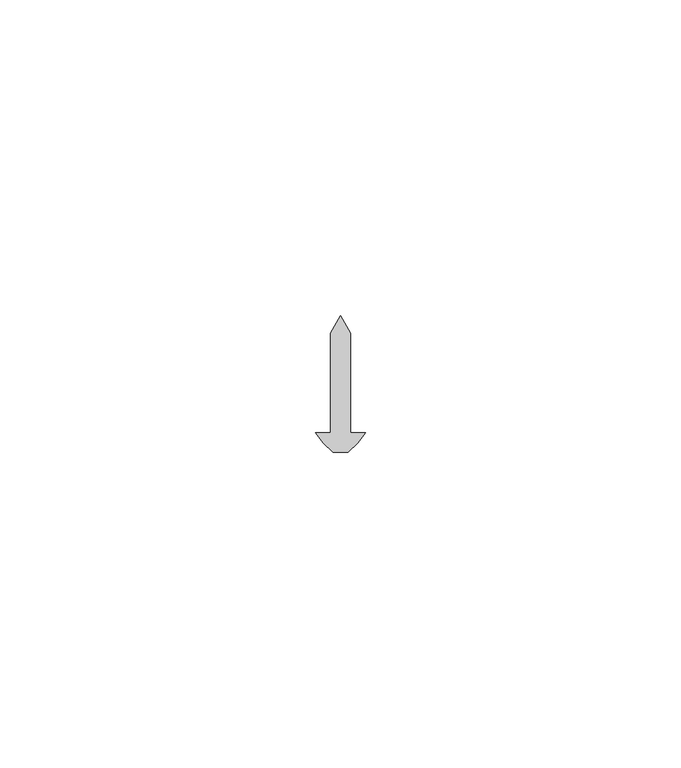
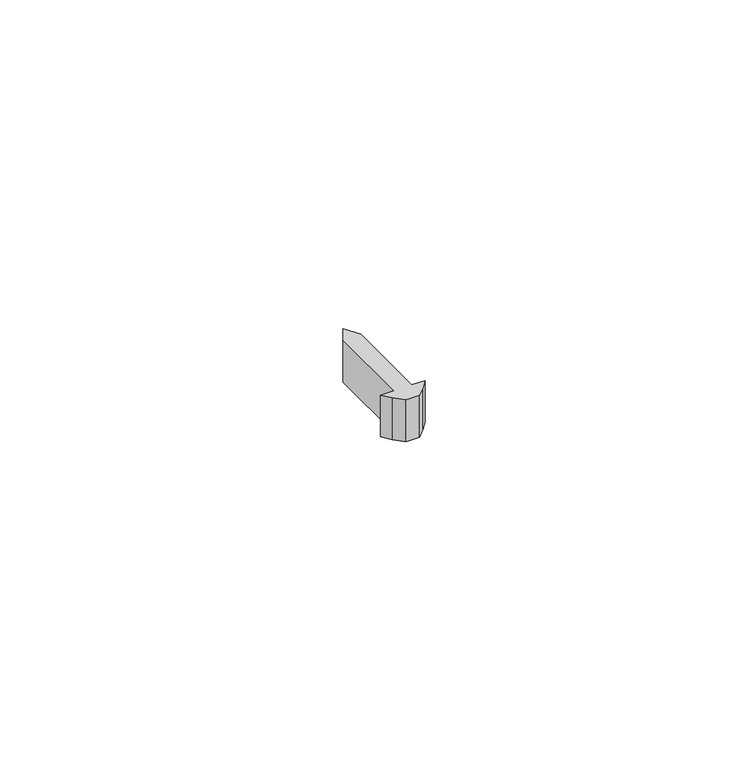
"""IFC4 building model written with IfcOpenShell, lengths in millimetres: proxy geometry, Generic Models 7:Generic Models 1:3:Generic Models 1:3 : Generic Models 7:Generic Models 1:305549:3:Generic Models 1:3:Generic Models 1:3 : Generic Models 7:Generic Models 1:305549:3 : Generic Models 7:Generic Models 1:3:Generic Models 1:3 : Generic Models 7:Generic Models 1:305549:301244:19 : Generic Models 7:Generic Models 1:3:Generic Models 1:3 : Generic Models 7:Generic Models 1:305549:3:Generic Models 1:3:Generic Models 1:3 : Generic Models 7:Generic Models 1:305549:3 : Generic Models 7:Generic Models 1:3:Generic Models 1:3 : Generic Models 7:Generic Models 1:305549:301244:308848."""

from ifc_helpers import new_model, si_unit, frame, origin, place, context, project, spatial, polyline, outline, extrude, source, transform, mapped, element, save


def generic_models_55637cdd(model_context):
    return source(origin(), model_context, "Body", "SweptSolid", [
        extrude(outline(polyline([(594996.9742239, -579084.8288841), (594999.3554739, -579084.8288841), (594998.1372784, -579086.3559421), (594996.5853882, -579087.9078323), (594994.1880597, -579087.9078323), (594992.6361695, -579086.3559421), (594991.4179739, -579084.8288841), (594993.7992239, -579084.8288841), (594993.7992239, -579069.0196286), (594995.3867239, -579066.2699979), (594996.9742239, -579069.0196286), (594996.9742239, -579084.8288841)])), frame((0.0, 0.0, 1237.45625), z_axis=(0.0, 0.0, 1.0), x_axis=(1.0, 0.0, 0.0)), (0.0, 0.0, 1.0), 7.9375),
    ])


if __name__ == "__main__":
    model = new_model("IFC4")
    model_context = context("Model", 3, world=origin())
    ifc_project = project(units=[si_unit("LENGTHUNIT", "METRE", prefix="MILLI")], contexts=[model_context])
    site = spatial("IfcSite", under=ifc_project)
    building = spatial("IfcBuilding", under=site)
    placement = place(None, origin())
    generic_models_shape = generic_models_55637cdd(model_context)
    element("IfcBuildingElementProxy", 1, Name="Generic Models 7:Generic Models 1:3:Generic Models 1:3 : Generic Models 7:Generic Models 1:305549:3:Generic Models 1:3:Generic Models 1:3 : Generic Models 7:Generic Models 1:305549:3 : Generic Models 7:Generic Models 1:3:Generic Models 1:3 : Generic Models 7:Generic Models 1:305549:301244:19 : Generic Models 7:Generic Models 1:3:Generic Models 1:3 : Generic Models 7:Generic Models 1:305549:3:Generic Models 1:3:Generic Models 1:3 : Generic Models 7:Generic Models 1:305549:3 : Generic Models 7:Generic Models 1:3:Generic Models 1:3 : Generic Models 7:Generic Models 1:305549:301244:308848", ObjectType="Generic Models 7:Generic Models 1:3:Generic Models 1:3 : Generic Models 7:Generic Models 1:305549:3:Generic Models 1:3:Generic Models 1:3 : Generic Models 7:Generic Models 1:305549:3 : Generic Models 7:Generic Models 1:3:Generic Models 1:3 : Generic Models 7:Generic Models 1:305549:301244:19 : Generic Models 7:Generic Models 1:3:Generic Models 1:3 : Generic Models 7:Generic Models 1:305549:3:Generic Models 1:3:Generic Models 1:3 : Generic Models 7:Generic Models 1:305549:3 : Generic Models 7:Generic Models 1:3:Generic Models 1:3 : Generic Models 7:Generic Models 1:305549:301244:308848", at=placement, inside=building, context=model_context, shape_type="MappedRepresentation", body=[
        mapped(generic_models_shape, transform((0.0, 0.0, 0.0), x_axis=(1.0, 0.0, 0.0), y_axis=(0.0, 1.0, 0.0), z_axis=(0.0, 0.0, 1.0))),
    ])
    save(model, "model.ifc")

# Revit data of these elements
# Type "Generic Models 7:Generic Models 1:3:Generic Models 1:3 : Generic Models 7:Generic Models 1:305549:3:Generic Models 1:3:Generic Models 1:3 : Generic Models 7:Generic Models 1:305549:3 : Generic Models 7:Generic Models 1:3:Generic Models 1:3 : Generic Models 7:Generic Models 1:305549:301244:19 : Generic Models 7:Generic Models 1:3:Generic Models 1:3 : Generic Models 7:Generic Models 1:305549:3:Generic Models 1:3:Generic Models 1:3 : Generic Models 7:Generic Models 1:305549:3 : Generic Models 7:Generic Models 1:3:Generic Models 1:3 : Generic Models 7:Generic Models 1:305549:301244:308848"
#   NameOverride = "Generic Models 7:Generic Models 1:3:Generic Models 1:3 : Generic Models 7:Generic Models 1:305549:3:Generic Models 1:3:Generic Models 1:3 : Generic Models 7:Generic Models 1:305549:3 : Generic Models 7:Generic Models 1:3:Generic Models 1:3 : Generic Models 7:Generic Models 1:305549:301244:308848"
#   ObjectTypeOverride = "Generic Models 1:3:Generic Models 1:3 : Generic Models 7:Generic Models 1:305549:3 : Generic Models 7:Generic Models 1:3:Generic Models 1:3 : Generic Models 7:Generic Models 1:305549:301244"
#   Reference = "Generic Models 1"
#   Tag = "308848"
# Element 1 (IfcBuildingElementProxy, "Generic Models 7:Generic Models 1:3:Generic Models 1:3 : Generic Models 7:Generic Models 1:305549:3:Generic Models 1:3:Generic Models 1:3 : Generic Models 7:Generic Models 1:305549:3 : Generic Models 7:Generic Models 1:3:Generic Models 1:3 : Generic Models 7:Generic Models 1:305549:301244:19 : Generic Models 7:Generic Models 1:3:Generic Models 1:3 : Generic Models 7:Generic Models 1:305549:3:Generic Models 1:3:Generic Models 1:3 : Generic Models 7:Generic Models 1:305549:3 : Generic Models 7:Generic Models 1:3:Generic Models 1:3 : Generic Models 7:Generic Models 1:305549:301244:308848")
#   Materials on its faces: "FASTENERS (T.B.D)"
# Materials
#   "FASTENERS (T.B.D)": class "Generic", colour RGB 120 120 120, transparency 0, Cost = 0
